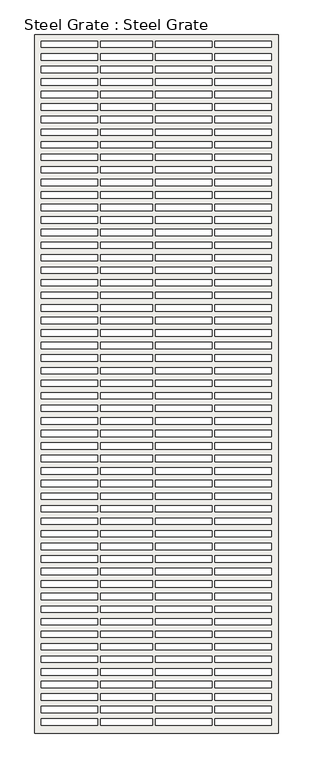
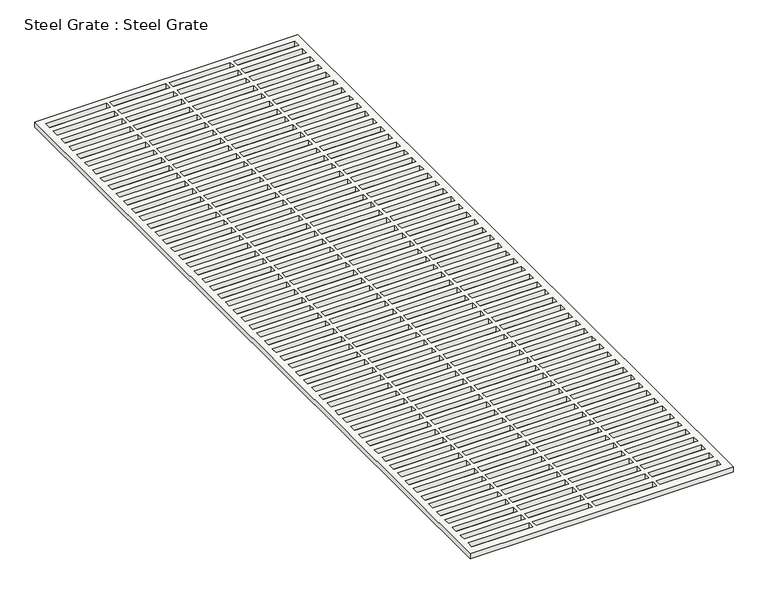
"""IFC4 building model written with IfcOpenShell, lengths in millimetres: slab geometry, Steel Grate : Steel Grate."""

from ifc_helpers import new_model, si_unit, frame, origin, place, context, project, spatial, polyline, outline, extrude, source, transform, mapped, element, save


def steel_grate_steel_grate_db4f937c(model_context):
    return source(origin(), model_context, "Body", "SweptSolid", [
        extrude(outline(polyline([(-85378.6917117, 6578.6), (-85378.6917117, 927.1), (-87350.6, 927.1), (-87350.6, 6578.6), (-85378.6917117, 6578.6)]), holes=[polyline([(-86842.6, 6527.8), (-87299.8, 6527.8), (-87299.8, 6477.0), (-86842.6, 6477.0), (-86842.6, 6527.8)]), polyline([(-85432.9, 6527.8), (-85890.1, 6527.8), (-85890.1, 6477.0), (-85432.9, 6477.0), (-85432.9, 6527.8)]), polyline([(-85915.5, 6527.8), (-86372.7, 6527.8), (-86372.7, 6477.0), (-85915.5, 6477.0), (-85915.5, 6527.8)]), polyline([(-86817.2, 6477.0), (-86398.1, 6477.0), (-86398.1, 6527.8), (-86817.2, 6527.8), (-86817.2, 6477.0)]), polyline([(-86842.6, 6426.2), (-87299.8, 6426.2), (-87299.8, 6375.4), (-86842.6, 6375.4), (-86842.6, 6426.2)]), polyline([(-85432.9, 6426.2), (-85890.1, 6426.2), (-85890.1, 6375.4), (-85432.9, 6375.4), (-85432.9, 6426.2)]), polyline([(-85915.5, 6426.2), (-86372.7, 6426.2), (-86372.7, 6375.4), (-85915.5, 6375.4), (-85915.5, 6426.2)]), polyline([(-86817.2, 6375.4), (-86398.1, 6375.4), (-86398.1, 6426.2), (-86817.2, 6426.2), (-86817.2, 6375.4)]), polyline([(-86842.6, 6324.6), (-87299.8, 6324.6), (-87299.8, 6273.8), (-86842.6, 6273.8), (-86842.6, 6324.6)]), polyline([(-85432.9, 6324.6), (-85890.1, 6324.6), (-85890.1, 6273.8), (-85432.9, 6273.8), (-85432.9, 6324.6)]), polyline([(-85915.5, 6324.6), (-86372.7, 6324.6), (-86372.7, 6273.8), (-85915.5, 6273.8), (-85915.5, 6324.6)]), polyline([(-86817.2, 6273.8), (-86398.1, 6273.8), (-86398.1, 6324.6), (-86817.2, 6324.6), (-86817.2, 6273.8)]), polyline([(-86842.6, 6223.0), (-87299.8, 6223.0), (-87299.8, 6172.2), (-86842.6, 6172.2), (-86842.6, 6223.0)]), polyline([(-85432.9, 6223.0), (-85890.1, 6223.0), (-85890.1, 6172.2), (-85432.9, 6172.2), (-85432.9, 6223.0)]), polyline([(-85915.5, 6223.0), (-86372.7, 6223.0), (-86372.7, 6172.2), (-85915.5, 6172.2), (-85915.5, 6223.0)]), polyline([(-86817.2, 6172.2), (-86398.1, 6172.2), (-86398.1, 6223.0), (-86817.2, 6223.0), (-86817.2, 6172.2)]), polyline([(-86842.6, 6121.4), (-87299.8, 6121.4), (-87299.8, 6070.6), (-86842.6, 6070.6), (-86842.6, 6121.4)]), polyline([(-85432.9, 6121.4), (-85890.1, 6121.4), (-85890.1, 6070.6), (-85432.9, 6070.6), (-85432.9, 6121.4)]), polyline([(-85915.5, 6121.4), (-86372.7, 6121.4), (-86372.7, 6070.6), (-85915.5, 6070.6), (-85915.5, 6121.4)]), polyline([(-86817.2, 6070.6), (-86398.1, 6070.6), (-86398.1, 6121.4), (-86817.2, 6121.4), (-86817.2, 6070.6)]), polyline([(-86842.6, 6019.8), (-87299.8, 6019.8), (-87299.8, 5969.0), (-86842.6, 5969.0), (-86842.6, 6019.8)]), polyline([(-85432.9, 6019.8), (-85890.1, 6019.8), (-85890.1, 5969.0), (-85432.9, 5969.0), (-85432.9, 6019.8)]), polyline([(-85915.5, 6019.8), (-86372.7, 6019.8), (-86372.7, 5969.0), (-85915.5, 5969.0), (-85915.5, 6019.8)]), polyline([(-86817.2, 5969.0), (-86398.1, 5969.0), (-86398.1, 6019.8), (-86817.2, 6019.8), (-86817.2, 5969.0)]), polyline([(-86842.6, 5918.2), (-87299.8, 5918.2), (-87299.8, 5867.4), (-86842.6, 5867.4), (-86842.6, 5918.2)]), polyline([(-85432.9, 5918.2), (-85890.1, 5918.2), (-85890.1, 5867.4), (-85432.9, 5867.4), (-85432.9, 5918.2)]), polyline([(-85915.5, 5918.2), (-86372.7, 5918.2), (-86372.7, 5867.4), (-85915.5, 5867.4), (-85915.5, 5918.2)]), polyline([(-86817.2, 5867.4), (-86398.1, 5867.4), (-86398.1, 5918.2), (-86817.2, 5918.2), (-86817.2, 5867.4)]), polyline([(-86842.6, 5816.6), (-87299.8, 5816.6), (-87299.8, 5765.8), (-86842.6, 5765.8), (-86842.6, 5816.6)]), polyline([(-85432.9, 5816.6), (-85890.1, 5816.6), (-85890.1, 5765.8), (-85432.9, 5765.8), (-85432.9, 5816.6)]), polyline([(-85915.5, 5816.6), (-86372.7, 5816.6), (-86372.7, 5765.8), (-85915.5, 5765.8), (-85915.5, 5816.6)]), polyline([(-86817.2, 5765.8), (-86398.1, 5765.8), (-86398.1, 5816.6), (-86817.2, 5816.6), (-86817.2, 5765.8)]), polyline([(-86842.6, 5715.0), (-87299.8, 5715.0), (-87299.8, 5664.2), (-86842.6, 5664.2), (-86842.6, 5715.0)]), polyline([(-85432.9, 5715.0), (-85890.1, 5715.0), (-85890.1, 5664.2), (-85432.9, 5664.2), (-85432.9, 5715.0)]), polyline([(-85915.5, 5715.0), (-86372.7, 5715.0), (-86372.7, 5664.2), (-85915.5, 5664.2), (-85915.5, 5715.0)]), polyline([(-86817.2, 5664.2), (-86398.1, 5664.2), (-86398.1, 5715.0), (-86817.2, 5715.0), (-86817.2, 5664.2)]), polyline([(-86842.6, 5613.4), (-87299.8, 5613.4), (-87299.8, 5562.6), (-86842.6, 5562.6), (-86842.6, 5613.4)]), polyline([(-85432.9, 5613.4), (-85890.1, 5613.4), (-85890.1, 5562.6), (-85432.9, 5562.6), (-85432.9, 5613.4)]), polyline([(-85915.5, 5613.4), (-86372.7, 5613.4), (-86372.7, 5562.6), (-85915.5, 5562.6), (-85915.5, 5613.4)]), polyline([(-86817.2, 5562.6), (-86398.1, 5562.6), (-86398.1, 5613.4), (-86817.2, 5613.4), (-86817.2, 5562.6)]), polyline([(-86842.6, 5511.8), (-87299.8, 5511.8), (-87299.8, 5461.0), (-86842.6, 5461.0), (-86842.6, 5511.8)]), polyline([(-85432.9, 5511.8), (-85890.1, 5511.8), (-85890.1, 5461.0), (-85432.9, 5461.0), (-85432.9, 5511.8)]), polyline([(-85915.5, 5511.8), (-86372.7, 5511.8), (-86372.7, 5461.0), (-85915.5, 5461.0), (-85915.5, 5511.8)]), polyline([(-86817.2, 5461.0), (-86398.1, 5461.0), (-86398.1, 5511.8), (-86817.2, 5511.8), (-86817.2, 5461.0)]), polyline([(-86842.6, 5410.2), (-87299.8, 5410.2), (-87299.8, 5359.4), (-86842.6, 5359.4), (-86842.6, 5410.2)]), polyline([(-85432.9, 5410.2), (-85890.1, 5410.2), (-85890.1, 5359.4), (-85432.9, 5359.4), (-85432.9, 5410.2)]), polyline([(-85915.5, 5410.2), (-86372.7, 5410.2), (-86372.7, 5359.4), (-85915.5, 5359.4), (-85915.5, 5410.2)]), polyline([(-86817.2, 5359.4), (-86398.1, 5359.4), (-86398.1, 5410.2), (-86817.2, 5410.2), (-86817.2, 5359.4)]), polyline([(-86842.6, 5308.6), (-87299.8, 5308.6), (-87299.8, 5257.8), (-86842.6, 5257.8), (-86842.6, 5308.6)]), polyline([(-85432.9, 5308.6), (-85890.1, 5308.6), (-85890.1, 5257.8), (-85432.9, 5257.8), (-85432.9, 5308.6)]), polyline([(-85915.5, 5308.6), (-86372.7, 5308.6), (-86372.7, 5257.8), (-85915.5, 5257.8), (-85915.5, 5308.6)]), polyline([(-86817.2, 5257.8), (-86398.1, 5257.8), (-86398.1, 5308.6), (-86817.2, 5308.6), (-86817.2, 5257.8)]), polyline([(-86842.6, 5207.0), (-87299.8, 5207.0), (-87299.8, 5156.2), (-86842.6, 5156.2), (-86842.6, 5207.0)]), polyline([(-85432.9, 5207.0), (-85890.1, 5207.0), (-85890.1, 5156.2), (-85432.9, 5156.2), (-85432.9, 5207.0)]), polyline([(-85915.5, 5207.0), (-86372.7, 5207.0), (-86372.7, 5156.2), (-85915.5, 5156.2), (-85915.5, 5207.0)]), polyline([(-86817.2, 5156.2), (-86398.1, 5156.2), (-86398.1, 5207.0), (-86817.2, 5207.0), (-86817.2, 5156.2)]), polyline([(-86842.6, 5105.4), (-87299.8, 5105.4), (-87299.8, 5054.6), (-86842.6, 5054.6), (-86842.6, 5105.4)]), polyline([(-85432.9, 5105.4), (-85890.1, 5105.4), (-85890.1, 5054.6), (-85432.9, 5054.6), (-85432.9, 5105.4)]), polyline([(-85915.5, 5105.4), (-86372.7, 5105.4), (-86372.7, 5054.6), (-85915.5, 5054.6), (-85915.5, 5105.4)]), polyline([(-86817.2, 5054.6), (-86398.1, 5054.6), (-86398.1, 5105.4), (-86817.2, 5105.4), (-86817.2, 5054.6)]), polyline([(-86842.6, 5003.8), (-87299.8, 5003.8), (-87299.8, 4953.0), (-86842.6, 4953.0), (-86842.6, 5003.8)]), polyline([(-85432.9, 5003.8), (-85890.1, 5003.8), (-85890.1, 4953.0), (-85432.9, 4953.0), (-85432.9, 5003.8)]), polyline([(-85915.5, 5003.8), (-86372.7, 5003.8), (-86372.7, 4953.0), (-85915.5, 4953.0), (-85915.5, 5003.8)]), polyline([(-86817.2, 4953.0), (-86398.1, 4953.0), (-86398.1, 5003.8), (-86817.2, 5003.8), (-86817.2, 4953.0)]), polyline([(-86842.6, 4902.2), (-87299.8, 4902.2), (-87299.8, 4851.4), (-86842.6, 4851.4), (-86842.6, 4902.2)]), polyline([(-85432.9, 4902.2), (-85890.1, 4902.2), (-85890.1, 4851.4), (-85432.9, 4851.4), (-85432.9, 4902.2)]), polyline([(-85915.5, 4902.2), (-86372.7, 4902.2), (-86372.7, 4851.4), (-85915.5, 4851.4), (-85915.5, 4902.2)]), polyline([(-86817.2, 4851.4), (-86398.1, 4851.4), (-86398.1, 4902.2), (-86817.2, 4902.2), (-86817.2, 4851.4)]), polyline([(-86842.6, 4800.6), (-87299.8, 4800.6), (-87299.8, 4749.8), (-86842.6, 4749.8), (-86842.6, 4800.6)]), polyline([(-85432.9, 4800.6), (-85890.1, 4800.6), (-85890.1, 4749.8), (-85432.9, 4749.8), (-85432.9, 4800.6)]), polyline([(-85915.5, 4800.6), (-86372.7, 4800.6), (-86372.7, 4749.8), (-85915.5, 4749.8), (-85915.5, 4800.6)]), polyline([(-86817.2, 4749.8), (-86398.1, 4749.8), (-86398.1, 4800.6), (-86817.2, 4800.6), (-86817.2, 4749.8)]), polyline([(-86842.6, 4699.0), (-87299.8, 4699.0), (-87299.8, 4648.2), (-86842.6, 4648.2), (-86842.6, 4699.0)]), polyline([(-85432.9, 4699.0), (-85890.1, 4699.0), (-85890.1, 4648.2), (-85432.9, 4648.2), (-85432.9, 4699.0)]), polyline([(-85915.5, 4699.0), (-86372.7, 4699.0), (-86372.7, 4648.2), (-85915.5, 4648.2), (-85915.5, 4699.0)]), polyline([(-86817.2, 4648.2), (-86398.1, 4648.2), (-86398.1, 4699.0), (-86817.2, 4699.0), (-86817.2, 4648.2)]), polyline([(-86842.6, 4597.4), (-87299.8, 4597.4), (-87299.8, 4546.6), (-86842.6, 4546.6), (-86842.6, 4597.4)]), polyline([(-85432.9, 4597.4), (-85890.1, 4597.4), (-85890.1, 4546.6), (-85432.9, 4546.6), (-85432.9, 4597.4)]), polyline([(-85915.5, 4597.4), (-86372.7, 4597.4), (-86372.7, 4546.6), (-85915.5, 4546.6), (-85915.5, 4597.4)]), polyline([(-86817.2, 4546.6), (-86398.1, 4546.6), (-86398.1, 4597.4), (-86817.2, 4597.4), (-86817.2, 4546.6)]), polyline([(-86842.6, 4495.8), (-87299.8, 4495.8), (-87299.8, 4445.0), (-86842.6, 4445.0), (-86842.6, 4495.8)]), polyline([(-85432.9, 4495.8), (-85890.1, 4495.8), (-85890.1, 4445.0), (-85432.9, 4445.0), (-85432.9, 4495.8)]), polyline([(-85915.5, 4495.8), (-86372.7, 4495.8), (-86372.7, 4445.0), (-85915.5, 4445.0), (-85915.5, 4495.8)]), polyline([(-86817.2, 4445.0), (-86398.1, 4445.0), (-86398.1, 4495.8), (-86817.2, 4495.8), (-86817.2, 4445.0)]), polyline([(-86842.6, 4394.2), (-87299.8, 4394.2), (-87299.8, 4343.4), (-86842.6, 4343.4), (-86842.6, 4394.2)]), polyline([(-85432.9, 4394.2), (-85890.1, 4394.2), (-85890.1, 4343.4), (-85432.9, 4343.4), (-85432.9, 4394.2)]), polyline([(-85915.5, 4394.2), (-86372.7, 4394.2), (-86372.7, 4343.4), (-85915.5, 4343.4), (-85915.5, 4394.2)]), polyline([(-86817.2, 4343.4), (-86398.1, 4343.4), (-86398.1, 4394.2), (-86817.2, 4394.2), (-86817.2, 4343.4)]), polyline([(-86842.6, 4292.6), (-87299.8, 4292.6), (-87299.8, 4241.8), (-86842.6, 4241.8), (-86842.6, 4292.6)]), polyline([(-85432.9, 4292.6), (-85890.1, 4292.6), (-85890.1, 4241.8), (-85432.9, 4241.8), (-85432.9, 4292.6)]), polyline([(-85915.5, 4292.6), (-86372.7, 4292.6), (-86372.7, 4241.8), (-85915.5, 4241.8), (-85915.5, 4292.6)]), polyline([(-86817.2, 4241.8), (-86398.1, 4241.8), (-86398.1, 4292.6), (-86817.2, 4292.6), (-86817.2, 4241.8)]), polyline([(-86842.6, 4191.0), (-87299.8, 4191.0), (-87299.8, 4140.2), (-86842.6, 4140.2), (-86842.6, 4191.0)]), polyline([(-85432.9, 4191.0), (-85890.1, 4191.0), (-85890.1, 4140.2), (-85432.9, 4140.2), (-85432.9, 4191.0)]), polyline([(-85915.5, 4191.0), (-86372.7, 4191.0), (-86372.7, 4140.2), (-85915.5, 4140.2), (-85915.5, 4191.0)]), polyline([(-86817.2, 4140.2), (-86398.1, 4140.2), (-86398.1, 4191.0), (-86817.2, 4191.0), (-86817.2, 4140.2)]), polyline([(-86842.6, 4089.4), (-87299.8, 4089.4), (-87299.8, 4038.6), (-86842.6, 4038.6), (-86842.6, 4089.4)]), polyline([(-85432.9, 4089.4), (-85890.1, 4089.4), (-85890.1, 4038.6), (-85432.9, 4038.6), (-85432.9, 4089.4)]), polyline([(-85915.5, 4089.4), (-86372.7, 4089.4), (-86372.7, 4038.6), (-85915.5, 4038.6), (-85915.5, 4089.4)]), polyline([(-86817.2, 4038.6), (-86398.1, 4038.6), (-86398.1, 4089.4), (-86817.2, 4089.4), (-86817.2, 4038.6)]), polyline([(-86842.6, 3987.8), (-87299.8, 3987.8), (-87299.8, 3937.0), (-86842.6, 3937.0), (-86842.6, 3987.8)]), polyline([(-85432.9, 3987.8), (-85890.1, 3987.8), (-85890.1, 3937.0), (-85432.9, 3937.0), (-85432.9, 3987.8)]), polyline([(-85915.5, 3987.8), (-86372.7, 3987.8), (-86372.7, 3937.0), (-85915.5, 3937.0), (-85915.5, 3987.8)]), polyline([(-86817.2, 3937.0), (-86398.1, 3937.0), (-86398.1, 3987.8), (-86817.2, 3987.8), (-86817.2, 3937.0)]), polyline([(-86842.6, 3886.2), (-87299.8, 3886.2), (-87299.8, 3835.4), (-86842.6, 3835.4), (-86842.6, 3886.2)]), polyline([(-85432.9, 3886.2), (-85890.1, 3886.2), (-85890.1, 3835.4), (-85432.9, 3835.4), (-85432.9, 3886.2)]), polyline([(-85915.5, 3886.2), (-86372.7, 3886.2), (-86372.7, 3835.4), (-85915.5, 3835.4), (-85915.5, 3886.2)]), polyline([(-86817.2, 3835.4), (-86398.1, 3835.4), (-86398.1, 3886.2), (-86817.2, 3886.2), (-86817.2, 3835.4)]), polyline([(-86842.6, 3784.6), (-87299.8, 3784.6), (-87299.8, 3733.8), (-86842.6, 3733.8), (-86842.6, 3784.6)]), polyline([(-85432.9, 3784.6), (-85890.1, 3784.6), (-85890.1, 3733.8), (-85432.9, 3733.8), (-85432.9, 3784.6)]), polyline([(-85915.5, 3784.6), (-86372.7, 3784.6), (-86372.7, 3733.8), (-85915.5, 3733.8), (-85915.5, 3784.6)]), polyline([(-86817.2, 3733.8), (-86398.1, 3733.8), (-86398.1, 3784.6), (-86817.2, 3784.6), (-86817.2, 3733.8)]), polyline([(-86842.6, 3683.0), (-87299.8, 3683.0), (-87299.8, 3632.2), (-86842.6, 3632.2), (-86842.6, 3683.0)]), polyline([(-85432.9, 3683.0), (-85890.1, 3683.0), (-85890.1, 3632.2), (-85432.9, 3632.2), (-85432.9, 3683.0)]), polyline([(-85915.5, 3683.0), (-86372.7, 3683.0), (-86372.7, 3632.2), (-85915.5, 3632.2), (-85915.5, 3683.0)]), polyline([(-86817.2, 3632.2), (-86398.1, 3632.2), (-86398.1, 3683.0), (-86817.2, 3683.0), (-86817.2, 3632.2)]), polyline([(-86842.6, 3581.4), (-87299.8, 3581.4), (-87299.8, 3530.6), (-86842.6, 3530.6), (-86842.6, 3581.4)]), polyline([(-85432.9, 3581.4), (-85890.1, 3581.4), (-85890.1, 3530.6), (-85432.9, 3530.6), (-85432.9, 3581.4)]), polyline([(-85915.5, 3581.4), (-86372.7, 3581.4), (-86372.7, 3530.6), (-85915.5, 3530.6), (-85915.5, 3581.4)]), polyline([(-86817.2, 3530.6), (-86398.1, 3530.6), (-86398.1, 3581.4), (-86817.2, 3581.4), (-86817.2, 3530.6)]), polyline([(-86842.6, 3479.8), (-87299.8, 3479.8), (-87299.8, 3429.0), (-86842.6, 3429.0), (-86842.6, 3479.8)]), polyline([(-85432.9, 3479.8), (-85890.1, 3479.8), (-85890.1, 3429.0), (-85432.9, 3429.0), (-85432.9, 3479.8)]), polyline([(-85915.5, 3479.8), (-86372.7, 3479.8), (-86372.7, 3429.0), (-85915.5, 3429.0), (-85915.5, 3479.8)]), polyline([(-86817.2, 3429.0), (-86398.1, 3429.0), (-86398.1, 3479.8), (-86817.2, 3479.8), (-86817.2, 3429.0)]), polyline([(-86842.6, 3378.2), (-87299.8, 3378.2), (-87299.8, 3327.4), (-86842.6, 3327.4), (-86842.6, 3378.2)]), polyline([(-85432.9, 3378.2), (-85890.1, 3378.2), (-85890.1, 3327.4), (-85432.9, 3327.4), (-85432.9, 3378.2)]), polyline([(-85915.5, 3378.2), (-86372.7, 3378.2), (-86372.7, 3327.4), (-85915.5, 3327.4), (-85915.5, 3378.2)]), polyline([(-86817.2, 3327.4), (-86398.1, 3327.4), (-86398.1, 3378.2), (-86817.2, 3378.2), (-86817.2, 3327.4)]), polyline([(-86842.6, 3276.6), (-87299.8, 3276.6), (-87299.8, 3225.8), (-86842.6, 3225.8), (-86842.6, 3276.6)]), polyline([(-85432.9, 3276.6), (-85890.1, 3276.6), (-85890.1, 3225.8), (-85432.9, 3225.8), (-85432.9, 3276.6)]), polyline([(-85915.5, 3276.6), (-86372.7, 3276.6), (-86372.7, 3225.8), (-85915.5, 3225.8), (-85915.5, 3276.6)]), polyline([(-86817.2, 3225.8), (-86398.1, 3225.8), (-86398.1, 3276.6), (-86817.2, 3276.6), (-86817.2, 3225.8)]), polyline([(-86842.6, 3175.0), (-87299.8, 3175.0), (-87299.8, 3124.2), (-86842.6, 3124.2), (-86842.6, 3175.0)]), polyline([(-85432.9, 3175.0), (-85890.1, 3175.0), (-85890.1, 3124.2), (-85432.9, 3124.2), (-85432.9, 3175.0)]), polyline([(-85915.5, 3175.0), (-86372.7, 3175.0), (-86372.7, 3124.2), (-85915.5, 3124.2), (-85915.5, 3175.0)]), polyline([(-86817.2, 3124.2), (-86398.1, 3124.2), (-86398.1, 3175.0), (-86817.2, 3175.0), (-86817.2, 3124.2)]), polyline([(-86842.6, 3073.4), (-87299.8, 3073.4), (-87299.8, 3022.6), (-86842.6, 3022.6), (-86842.6, 3073.4)]), polyline([(-85432.9, 3073.4), (-85890.1, 3073.4), (-85890.1, 3022.6), (-85432.9, 3022.6), (-85432.9, 3073.4)]), polyline([(-85915.5, 3073.4), (-86372.7, 3073.4), (-86372.7, 3022.6), (-85915.5, 3022.6), (-85915.5, 3073.4)]), polyline([(-86817.2, 3022.6), (-86398.1, 3022.6), (-86398.1, 3073.4), (-86817.2, 3073.4), (-86817.2, 3022.6)]), polyline([(-86842.6, 2971.8), (-87299.8, 2971.8), (-87299.8, 2921.0), (-86842.6, 2921.0), (-86842.6, 2971.8)]), polyline([(-85432.9, 2971.8), (-85890.1, 2971.8), (-85890.1, 2921.0), (-85432.9, 2921.0), (-85432.9, 2971.8)]), polyline([(-85915.5, 2971.8), (-86372.7, 2971.8), (-86372.7, 2921.0), (-85915.5, 2921.0), (-85915.5, 2971.8)]), polyline([(-86817.2, 2921.0), (-86398.1, 2921.0), (-86398.1, 2971.8), (-86817.2, 2971.8), (-86817.2, 2921.0)]), polyline([(-86842.6, 2870.2), (-87299.8, 2870.2), (-87299.8, 2819.4), (-86842.6, 2819.4), (-86842.6, 2870.2)]), polyline([(-85432.9, 2870.2), (-85890.1, 2870.2), (-85890.1, 2819.4), (-85432.9, 2819.4), (-85432.9, 2870.2)]), polyline([(-85915.5, 2870.2), (-86372.7, 2870.2), (-86372.7, 2819.4), (-85915.5, 2819.4), (-85915.5, 2870.2)]), polyline([(-86817.2, 2819.4), (-86398.1, 2819.4), (-86398.1, 2870.2), (-86817.2, 2870.2), (-86817.2, 2819.4)]), polyline([(-86842.6, 2768.6), (-87299.8, 2768.6), (-87299.8, 2717.8), (-86842.6, 2717.8), (-86842.6, 2768.6)]), polyline([(-85432.9, 2768.6), (-85890.1, 2768.6), (-85890.1, 2717.8), (-85432.9, 2717.8), (-85432.9, 2768.6)]), polyline([(-85915.5, 2768.6), (-86372.7, 2768.6), (-86372.7, 2717.8), (-85915.5, 2717.8), (-85915.5, 2768.6)]), polyline([(-86817.2, 2717.8), (-86398.1, 2717.8), (-86398.1, 2768.6), (-86817.2, 2768.6), (-86817.2, 2717.8)]), polyline([(-86842.6, 2667.0), (-87299.8, 2667.0), (-87299.8, 2616.2), (-86842.6, 2616.2), (-86842.6, 2667.0)]), polyline([(-85432.9, 2667.0), (-85890.1, 2667.0), (-85890.1, 2616.2), (-85432.9, 2616.2), (-85432.9, 2667.0)]), polyline([(-85915.5, 2667.0), (-86372.7, 2667.0), (-86372.7, 2616.2), (-85915.5, 2616.2), (-85915.5, 2667.0)]), polyline([(-86817.2, 2616.2), (-86398.1, 2616.2), (-86398.1, 2667.0), (-86817.2, 2667.0), (-86817.2, 2616.2)]), polyline([(-86842.6, 2565.4), (-87299.8, 2565.4), (-87299.8, 2514.6), (-86842.6, 2514.6), (-86842.6, 2565.4)]), polyline([(-85432.9, 2565.4), (-85890.1, 2565.4), (-85890.1, 2514.6), (-85432.9, 2514.6), (-85432.9, 2565.4)]), polyline([(-85915.5, 2565.4), (-86372.7, 2565.4), (-86372.7, 2514.6), (-85915.5, 2514.6), (-85915.5, 2565.4)]), polyline([(-86817.2, 2514.6), (-86398.1, 2514.6), (-86398.1, 2565.4), (-86817.2, 2565.4), (-86817.2, 2514.6)]), polyline([(-86842.6, 2463.8), (-87299.8, 2463.8), (-87299.8, 2413.0), (-86842.6, 2413.0), (-86842.6, 2463.8)]), polyline([(-85432.9, 2463.8), (-85890.1, 2463.8), (-85890.1, 2413.0), (-85432.9, 2413.0), (-85432.9, 2463.8)]), polyline([(-85915.5, 2463.8), (-86372.7, 2463.8), (-86372.7, 2413.0), (-85915.5, 2413.0), (-85915.5, 2463.8)]), polyline([(-86817.2, 2413.0), (-86398.1, 2413.0), (-86398.1, 2463.8), (-86817.2, 2463.8), (-86817.2, 2413.0)]), polyline([(-86842.6, 2362.2), (-87299.8, 2362.2), (-87299.8, 2311.4), (-86842.6, 2311.4), (-86842.6, 2362.2)]), polyline([(-85432.9, 2362.2), (-85890.1, 2362.2), (-85890.1, 2311.4), (-85432.9, 2311.4), (-85432.9, 2362.2)]), polyline([(-85915.5, 2362.2), (-86372.7, 2362.2), (-86372.7, 2311.4), (-85915.5, 2311.4), (-85915.5, 2362.2)]), polyline([(-86817.2, 2311.4), (-86398.1, 2311.4), (-86398.1, 2362.2), (-86817.2, 2362.2), (-86817.2, 2311.4)]), polyline([(-86842.6, 2260.6), (-87299.8, 2260.6), (-87299.8, 2209.8), (-86842.6, 2209.8), (-86842.6, 2260.6)]), polyline([(-85432.9, 2260.6), (-85890.1, 2260.6), (-85890.1, 2209.8), (-85432.9, 2209.8), (-85432.9, 2260.6)]), polyline([(-85915.5, 2260.6), (-86372.7, 2260.6), (-86372.7, 2209.8), (-85915.5, 2209.8), (-85915.5, 2260.6)]), polyline([(-86817.2, 2209.8), (-86398.1, 2209.8), (-86398.1, 2260.6), (-86817.2, 2260.6), (-86817.2, 2209.8)]), polyline([(-86842.6, 2159.0), (-87299.8, 2159.0), (-87299.8, 2108.2), (-86842.6, 2108.2), (-86842.6, 2159.0)]), polyline([(-85432.9, 2159.0), (-85890.1, 2159.0), (-85890.1, 2108.2), (-85432.9, 2108.2), (-85432.9, 2159.0)]), polyline([(-85915.5, 2159.0), (-86372.7, 2159.0), (-86372.7, 2108.2), (-85915.5, 2108.2), (-85915.5, 2159.0)]), polyline([(-86817.2, 2108.2), (-86398.1, 2108.2), (-86398.1, 2159.0), (-86817.2, 2159.0), (-86817.2, 2108.2)]), polyline([(-86842.6, 2057.4), (-87299.8, 2057.4), (-87299.8, 2006.6), (-86842.6, 2006.6), (-86842.6, 2057.4)]), polyline([(-85432.9, 2057.4), (-85890.1, 2057.4), (-85890.1, 2006.6), (-85432.9, 2006.6), (-85432.9, 2057.4)]), polyline([(-85915.5, 2057.4), (-86372.7, 2057.4), (-86372.7, 2006.6), (-85915.5, 2006.6), (-85915.5, 2057.4)]), polyline([(-86817.2, 2006.6), (-86398.1, 2006.6), (-86398.1, 2057.4), (-86817.2, 2057.4), (-86817.2, 2006.6)]), polyline([(-86842.6, 1955.8), (-87299.8, 1955.8), (-87299.8, 1905.0), (-86842.6, 1905.0), (-86842.6, 1955.8)]), polyline([(-85432.9, 1955.8), (-85890.1, 1955.8), (-85890.1, 1905.0), (-85432.9, 1905.0), (-85432.9, 1955.8)]), polyline([(-85915.5, 1955.8), (-86372.7, 1955.8), (-86372.7, 1905.0), (-85915.5, 1905.0), (-85915.5, 1955.8)]), polyline([(-86817.2, 1905.0), (-86398.1, 1905.0), (-86398.1, 1955.8), (-86817.2, 1955.8), (-86817.2, 1905.0)]), polyline([(-86842.6, 1854.2), (-87299.8, 1854.2), (-87299.8, 1803.4), (-86842.6, 1803.4), (-86842.6, 1854.2)]), polyline([(-85432.9, 1854.2), (-85890.1, 1854.2), (-85890.1, 1803.4), (-85432.9, 1803.4), (-85432.9, 1854.2)]), polyline([(-85915.5, 1854.2), (-86372.7, 1854.2), (-86372.7, 1803.4), (-85915.5, 1803.4), (-85915.5, 1854.2)]), polyline([(-86817.2, 1803.4), (-86398.1, 1803.4), (-86398.1, 1854.2), (-86817.2, 1854.2), (-86817.2, 1803.4)]), polyline([(-86842.6, 1752.6), (-87299.8, 1752.6), (-87299.8, 1701.8), (-86842.6, 1701.8), (-86842.6, 1752.6)]), polyline([(-85432.9, 1752.6), (-85890.1, 1752.6), (-85890.1, 1701.8), (-85432.9, 1701.8), (-85432.9, 1752.6)]), polyline([(-85915.5, 1752.6), (-86372.7, 1752.6), (-86372.7, 1701.8), (-85915.5, 1701.8), (-85915.5, 1752.6)]), polyline([(-86817.2, 1701.8), (-86398.1, 1701.8), (-86398.1, 1752.6), (-86817.2, 1752.6), (-86817.2, 1701.8)]), polyline([(-86842.6, 1651.0), (-87299.8, 1651.0), (-87299.8, 1600.2), (-86842.6, 1600.2), (-86842.6, 1651.0)]), polyline([(-85432.9, 1651.0), (-85890.1, 1651.0), (-85890.1, 1600.2), (-85432.9, 1600.2), (-85432.9, 1651.0)]), polyline([(-85915.5, 1651.0), (-86372.7, 1651.0), (-86372.7, 1600.2), (-85915.5, 1600.2), (-85915.5, 1651.0)]), polyline([(-86817.2, 1600.2), (-86398.1, 1600.2), (-86398.1, 1651.0), (-86817.2, 1651.0), (-86817.2, 1600.2)]), polyline([(-86842.6, 1549.4), (-87299.8, 1549.4), (-87299.8, 1498.6), (-86842.6, 1498.6), (-86842.6, 1549.4)]), polyline([(-85432.9, 1549.4), (-85890.1, 1549.4), (-85890.1, 1498.6), (-85432.9, 1498.6), (-85432.9, 1549.4)]), polyline([(-85915.5, 1549.4), (-86372.7, 1549.4), (-86372.7, 1498.6), (-85915.5, 1498.6), (-85915.5, 1549.4)]), polyline([(-86817.2, 1498.6), (-86398.1, 1498.6), (-86398.1, 1549.4), (-86817.2, 1549.4), (-86817.2, 1498.6)]), polyline([(-86842.6, 1447.8), (-87299.8, 1447.8), (-87299.8, 1397.0), (-86842.6, 1397.0), (-86842.6, 1447.8)]), polyline([(-85432.9, 1447.8), (-85890.1, 1447.8), (-85890.1, 1397.0), (-85432.9, 1397.0), (-85432.9, 1447.8)]), polyline([(-85915.5, 1447.8), (-86372.7, 1447.8), (-86372.7, 1397.0), (-85915.5, 1397.0), (-85915.5, 1447.8)]), polyline([(-86817.2, 1397.0), (-86398.1, 1397.0), (-86398.1, 1447.8), (-86817.2, 1447.8), (-86817.2, 1397.0)]), polyline([(-86842.6, 1346.2), (-87299.8, 1346.2), (-87299.8, 1295.4), (-86842.6, 1295.4), (-86842.6, 1346.2)]), polyline([(-85432.9, 1346.2), (-85890.1, 1346.2), (-85890.1, 1295.4), (-85432.9, 1295.4), (-85432.9, 1346.2)]), polyline([(-85915.5, 1346.2), (-86372.7, 1346.2), (-86372.7, 1295.4), (-85915.5, 1295.4), (-85915.5, 1346.2)]), polyline([(-86817.2, 1295.4), (-86398.1, 1295.4), (-86398.1, 1346.2), (-86817.2, 1346.2), (-86817.2, 1295.4)]), polyline([(-86842.6, 1244.6), (-87299.8, 1244.6), (-87299.8, 1193.8), (-86842.6, 1193.8), (-86842.6, 1244.6)]), polyline([(-85432.9, 1244.6), (-85890.1, 1244.6), (-85890.1, 1193.8), (-85432.9, 1193.8), (-85432.9, 1244.6)]), polyline([(-85915.5, 1244.6), (-86372.7, 1244.6), (-86372.7, 1193.8), (-85915.5, 1193.8), (-85915.5, 1244.6)]), polyline([(-86817.2, 1193.8), (-86398.1, 1193.8), (-86398.1, 1244.6), (-86817.2, 1244.6), (-86817.2, 1193.8)]), polyline([(-86842.6, 1143.0), (-87299.8, 1143.0), (-87299.8, 1092.2), (-86842.6, 1092.2), (-86842.6, 1143.0)]), polyline([(-85432.9, 1143.0), (-85890.1, 1143.0), (-85890.1, 1092.2), (-85432.9, 1092.2), (-85432.9, 1143.0)]), polyline([(-85915.5, 1143.0), (-86372.7, 1143.0), (-86372.7, 1092.2), (-85915.5, 1092.2), (-85915.5, 1143.0)]), polyline([(-86817.2, 1092.2), (-86398.1, 1092.2), (-86398.1, 1143.0), (-86817.2, 1143.0), (-86817.2, 1092.2)]), polyline([(-86842.6, 1041.4), (-87299.8, 1041.4), (-87299.8, 990.6), (-86842.6, 990.6), (-86842.6, 1041.4)]), polyline([(-85432.9, 1041.4), (-85890.1, 1041.4), (-85890.1, 990.6), (-85432.9, 990.6), (-85432.9, 1041.4)]), polyline([(-85915.5, 1041.4), (-86372.7, 1041.4), (-86372.7, 990.6), (-85915.5, 990.6), (-85915.5, 1041.4)]), polyline([(-86817.2, 990.6), (-86398.1, 990.6), (-86398.1, 1041.4), (-86817.2, 1041.4), (-86817.2, 990.6)])]), frame((0.0, 0.0, 13034.1086008), z_axis=(0.0, 0.0, 1.0), x_axis=(1.0, 0.0, 0.0)), (0.0, 0.0, 1.0), 40.5413992),
    ])


if __name__ == "__main__":
    model = new_model("IFC4")
    model_context = context("Model", 3, world=origin())
    ifc_project = project(units=[si_unit("LENGTHUNIT", "METRE", prefix="MILLI")], contexts=[model_context])
    site = spatial("IfcSite", under=ifc_project)
    building = spatial("IfcBuilding", under=site)
    placement = place(None, origin())
    steel_grate_steel_grate_shape = steel_grate_steel_grate_db4f937c(model_context)
    element("IfcSlab", 1, ObjectType="Steel Grate : Steel Grate", at=placement, inside=building, context=model_context, shape_type="MappedRepresentation", body=[
        mapped(steel_grate_steel_grate_shape, transform((0.0, 0.0, 0.0), x_axis=(1.0, 0.0, 0.0), y_axis=(0.0, 1.0, 0.0), z_axis=(0.0, 0.0, 1.0))),
    ])
    save(model, "model.ifc")
